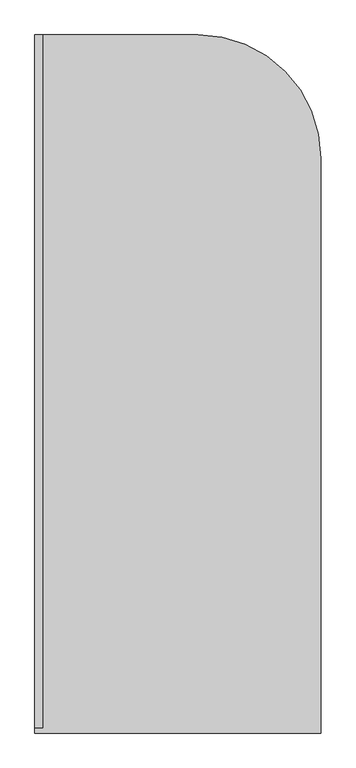
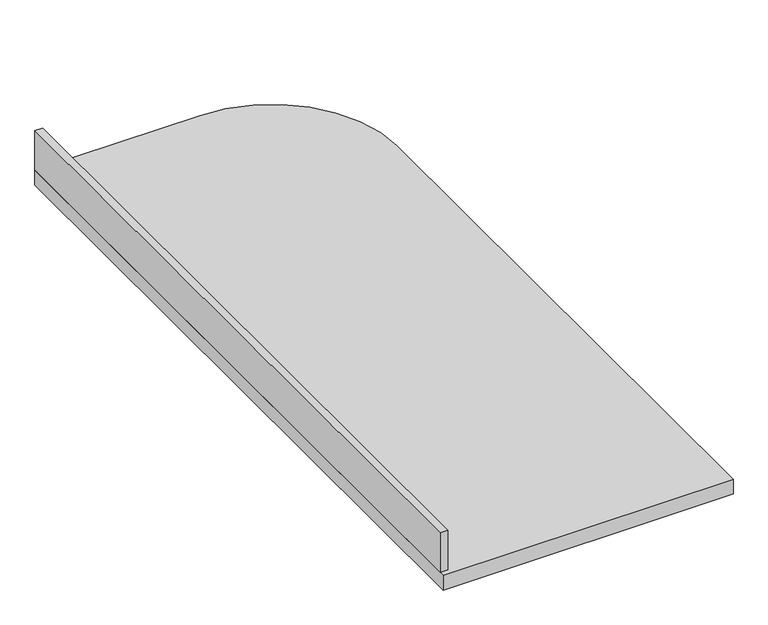
"""IFC4 building model written with IfcOpenShell, lengths in millimetres: furniture geometry, Kitchen - Baking counter : Kitchen - Baking counter."""

import ifcopenshell
import ifcopenshell.guid

model = None  # the IFC model being written
_history = None  # IfcOwnerHistory: only IFC2X3 demands one
_inside = {}  # id of a spatial element -> (the spatial element, [elements in it])
_under = {}  # id of a project, library or spatial element -> (it, [spatial elements below it])
_declared = {}  # id of a project -> (the project, [libraries it declares])
_typed = {}  # id of a type object -> (the type object, [elements of that type])
_made_of = {}  # id of a material, layer set ... -> (it, [elements and type objects made of it])


def new_model(schema):
    """Start an empty IFC model of exactly this schema.

    Asked for "IFC4X3", IfcOpenShell would pick the latest addendum, in which some entities
    have other attributes; the version numbers below select the first issue.
    IFC2X3 requires an IfcOwnerHistory on every rooted entity: one is made here for all.
    """
    global model, _history
    if schema == "IFC4X3":
        model = ifcopenshell.file(schema_version=(4, 3, 0, 0))
    else:
        model = ifcopenshell.file(schema=schema)
    _inside.clear()
    _under.clear()
    _declared.clear()
    _typed.clear()
    _made_of.clear()
    _history = None
    if model.schema == "IFC2X3":
        org = make("IfcOrganization", Name="unknown")
        user = make(
            "IfcPersonAndOrganization",
            ThePerson=make("IfcPerson", FamilyName="unknown"),
            TheOrganization=org,
        )
        app = make(
            "IfcApplication",
            ApplicationDeveloper=org,
            Version="unknown",
            ApplicationFullName="unknown",
            ApplicationIdentifier="unknown",
        )
        _history = make(
            "IfcOwnerHistory",
            OwningUser=user,
            OwningApplication=app,
            ChangeAction="ADDED",
            CreationDate=0,
        )
    return model


def make(cls, **values):
    """One entity of the class cls with the attributes given. An attribute that is None is left unset."""
    return model.create_entity(
        cls, **{name: value for name, value in values.items() if value is not None}
    )


def rooted(cls, **values):
    """An entity with a GlobalId (a new one), such as an element, a storey or a relation."""
    return make(cls, GlobalId=ifcopenshell.guid.new(), OwnerHistory=_history, **values)


def si_unit(unit_type, name, prefix=None):
    """IfcSIUnit, for example si_unit("LENGTHUNIT", "METRE", prefix="MILLI")."""
    return make("IfcSIUnit", UnitType=unit_type, Prefix=prefix, Name=name)


def assignment(units):
    """IfcUnitAssignment: the units of a project."""
    return None if units is None else make("IfcUnitAssignment", Units=units)


def point(xyz):
    """IfcCartesianPoint."""
    return None if xyz is None else make("IfcCartesianPoint", Coordinates=xyz)


def direction(xyz):
    """IfcDirection."""
    return None if xyz is None else make("IfcDirection", DirectionRatios=xyz)


def frame(location, z_axis=None, x_axis=None):
    """IfcAxis2Placement3D, a coordinate frame: its origin and axes. An axis left out is left unset."""
    return make(
        "IfcAxis2Placement3D",
        Location=point(location),
        Axis=direction(z_axis),
        RefDirection=direction(x_axis),
    )


def frame_2d(location, x_axis=None):
    """IfcAxis2Placement2D, a coordinate frame in the plane: its origin and x axis."""
    return make(
        "IfcAxis2Placement2D", Location=point(location), RefDirection=direction(x_axis)
    )


def origin():
    """The frame at (0, 0, 0) with its axes left unset."""
    return frame((0.0, 0.0, 0.0))


def place(relative_to, where):
    """IfcLocalPlacement: puts the frame where relative to a parent placement (None: the world)."""
    return make(
        "IfcLocalPlacement", PlacementRelTo=relative_to, RelativePlacement=where
    )


def context(
    kind, dimensions, precision=None, world=None, true_north=None, identifier=None
):
    """IfcGeometricRepresentationContext, for example the 3D "Model" context."""
    return make(
        "IfcGeometricRepresentationContext",
        ContextIdentifier=identifier,
        ContextType=kind,
        CoordinateSpaceDimension=dimensions,
        Precision=precision,
        WorldCoordinateSystem=world,
        TrueNorth=true_north,
    )


def project(units=None, contexts=None):
    """IfcProject with its units and contexts."""
    return rooted(
        "IfcProject",
        Name="project",
        RepresentationContexts=contexts,
        UnitsInContext=assignment(units),
    )


def spatial(cls, under=None, at=None, **own):
    """A site, building, storey or space (cls), placed at a placement, below another one or the project."""
    s = rooted(cls, ObjectPlacement=at, **own)
    if under is not None:
        _under.setdefault(under.id(), (under, []))[1].append(s)
    return s


def polyline(points):
    """IfcPolyline through the points."""
    return make("IfcPolyline", Points=[point(p) for p in points])


def circle_curve(where, radius):
    """IfcCircle in the frame where."""
    return make("IfcCircle", Position=where, Radius=radius)


def trimmed(basis, trim1, trim2, sense, master):
    """IfcTrimmedCurve: the piece of a basis curve between two trims."""
    return make(
        "IfcTrimmedCurve",
        BasisCurve=basis,
        Trim1=trim1,
        Trim2=trim2,
        SenseAgreement=sense,
        MasterRepresentation=master,
    )


def segment(curve, same_sense, transition):
    """IfcCompositeCurveSegment."""
    return make(
        "IfcCompositeCurveSegment",
        Transition=transition,
        SameSense=same_sense,
        ParentCurve=curve,
    )


def composite_curve(segments, self_intersect=None):
    """IfcCompositeCurve: segments joined end to end."""
    return make("IfcCompositeCurve", Segments=segments, SelfIntersect=self_intersect)


def outline(outer, holes=None, kind="AREA"):
    """IfcArbitraryClosedProfileDef: a profile drawn as a closed curve; with holes, ...WithVoids."""
    if holes is None:
        return make("IfcArbitraryClosedProfileDef", ProfileType=kind, OuterCurve=outer)
    return make(
        "IfcArbitraryProfileDefWithVoids",
        ProfileType=kind,
        OuterCurve=outer,
        InnerCurves=holes,
    )


def extrude(swept, where, along, depth):
    """IfcExtrudedAreaSolid: the profile swept, set in the frame where, extruded along a direction by depth."""
    return make(
        "IfcExtrudedAreaSolid",
        SweptArea=swept,
        Position=where,
        ExtrudedDirection=direction(along),
        Depth=depth,
    )


def shape(context_of_items, identifier, shape_type, items):
    """IfcShapeRepresentation: the items that make up one representation, for example the "Body"."""
    return make(
        "IfcShapeRepresentation",
        ContextOfItems=context_of_items,
        RepresentationIdentifier=identifier,
        RepresentationType=shape_type,
        Items=items,
    )


def source(mapping_origin, context_of_items, identifier, shape_type, items):
    """IfcRepresentationMap: a shape defined once, which mapped items show again and again."""
    return make(
        "IfcRepresentationMap",
        MappingOrigin=mapping_origin,
        MappedRepresentation=shape(context_of_items, identifier, shape_type, items),
    )


def transform(
    local_origin,
    x_axis=None,
    y_axis=None,
    z_axis=None,
    scale=None,
    scale2=None,
    scale3=None,
    uniform=True,
):
    """IfcCartesianTransformationOperator3D, or its non-uniform kind. x_axis, y_axis, z_axis: its Axis1, 2, 3."""
    if uniform:
        return make(
            "IfcCartesianTransformationOperator3D",
            Axis1=direction(x_axis),
            Axis2=direction(y_axis),
            LocalOrigin=point(local_origin),
            Scale=scale,
            Axis3=direction(z_axis),
        )
    return make(
        "IfcCartesianTransformationOperator3DnonUniform",
        Axis1=direction(x_axis),
        Axis2=direction(y_axis),
        LocalOrigin=point(local_origin),
        Scale=scale,
        Axis3=direction(z_axis),
        Scale2=scale2,
        Scale3=scale3,
    )


def mapped(mapping_source, mapping_target):
    """IfcMappedItem: shows the shape of a source again, moved by a transform."""
    return make(
        "IfcMappedItem", MappingSource=mapping_source, MappingTarget=mapping_target
    )


def made_of(thing, what):
    """Note that an element or type object is made of a material, layer set ...; save() writes the relation."""
    if what is not None:
        _made_of.setdefault(what.id(), (what, []))[1].append(thing)
    return thing


def element(
    cls,
    number,
    at=None,
    inside=None,
    cuts=None,
    type_object=None,
    material=None,
    context=None,
    identifier="Body",
    shape_type=None,
    held_by="IfcProductDefinitionShape",
    body=None,
    shapes=None,
    **own,
):
    """One element of the class cls, such as IfcWall. Its Tag is "e" and its number.

    at: its placement. inside: the storey or other place that contains it. cuts: it is an
    opening in that element (IfcRelVoidsElement). A single representation is given by context,
    identifier, shape_type and body (its items); several are given by shapes. held_by: the class
    of the entity that holds the representations. save() writes the other relations.
    """
    e = rooted(cls, Tag="e%d" % number, ObjectPlacement=at, **own)
    if body is not None:
        shapes = [shape(context, identifier, shape_type, body)]
    if shapes is not None:
        e.Representation = make(held_by, Representations=shapes)
    if inside is not None:
        _inside.setdefault(inside.id(), (inside, []))[1].append(e)
    if cuts is not None:
        rooted(
            "IfcRelVoidsElement", RelatingBuildingElement=cuts, RelatedOpeningElement=e
        )
    if type_object is not None:
        _typed.setdefault(type_object.id(), (type_object, []))[1].append(e)
    return made_of(e, material)


def aggregate(whole, parts):
    """IfcRelAggregates: a whole, such as a stair, and the parts it consists of."""
    return rooted("IfcRelAggregates", RelatingObject=whole, RelatedObjects=parts)


def save(model, path):
    """Write the relations noted so far, then the file.

    IfcRelAggregates (storeys below a building ...), IfcRelContainedInSpatialStructure (elements
    in a storey), IfcRelDefinesByType, IfcRelAssociatesMaterial and IfcRelDeclares: one each for
    every whole, place, type object, material and project.
    """
    for whole, parts in _under.values():
        aggregate(whole, parts)
    for where, things in _inside.values():
        rooted(
            "IfcRelContainedInSpatialStructure",
            RelatedElements=things,
            RelatingStructure=where,
        )
    for kind, things in _typed.values():
        rooted("IfcRelDefinesByType", RelatedObjects=things, RelatingType=kind)
    for what, things in _made_of.values():
        rooted("IfcRelAssociatesMaterial", RelatedObjects=things, RelatingMaterial=what)
    for by, libraries in _declared.values():
        rooted("IfcRelDeclares", RelatingContext=by, RelatedDefinitions=libraries)
    model.write(path)


def furniture_77338e29(model_context):
    return source(origin(), model_context, "Body", "SweptSolid", [
        extrude(outline(polyline([(3765.55, 10655.3), (3765.55, 12369.8), (3784.6, 12369.8), (3784.6, 10655.3), (3765.55, 10655.3)])), frame((0.0, 0.0, 914.4), z_axis=(0.0, 0.0, 1.0), x_axis=(1.0, 0.0, 0.0)), (0.0, 0.0, 1.0), 101.6),
        extrude(outline(composite_curve([segment(polyline([(4474.1779098, 12065.0), (4474.1779098, 10642.6), (3765.55, 10642.6), (3765.55, 12369.8), (4169.3779098, 12369.8)]), True, "CONTINUOUS"), segment(trimmed(circle_curve(frame_2d((4169.3779098, 12065.0)), 304.8), [point((4169.3779098, 12369.8))], [point((4474.1779098, 12065.0))], False, "CARTESIAN"), True, "CONTINUOUS")], self_intersect=False)), frame((0.0, 0.0, 876.3), z_axis=(0.0, 0.0, 1.0), x_axis=(1.0, 0.0, 0.0)), (0.0, 0.0, 1.0), 38.1),
    ])


if __name__ == "__main__":
    model = new_model("IFC4")
    model_context = context("Model", 3, world=origin())
    ifc_project = project(units=[si_unit("LENGTHUNIT", "METRE", prefix="MILLI")], contexts=[model_context])
    site = spatial("IfcSite", under=ifc_project)
    building = spatial("IfcBuilding", under=site)
    placement = place(None, origin())
    furniture_shape = furniture_77338e29(model_context)
    element("IfcFurniture", 1, ObjectType="Kitchen - Baking counter : Kitchen - Baking counter", at=placement, inside=building, context=model_context, shape_type="MappedRepresentation", body=[
        mapped(furniture_shape, transform((0.0, 0.0, 0.0), x_axis=(1.0, 0.0, 0.0), y_axis=(0.0, 1.0, 0.0), z_axis=(0.0, 0.0, 1.0))),
    ])
    save(model, "model.ifc")

# Revit data of these elements
# Type "Kitchen - Baking counter : Kitchen - Baking counter"
#   COBie.Type = no
# Element 1 (IfcFurniture, "Kitchen - Baking counter : Kitchen - Baking counter")
#   Materials on its faces: "Corian - Dusk"
# Materials
#   "Corian - Dusk": class "Plastic", colour RGB 75 95 146, transparency 0, Manufacturer = "Corning", Cost = 0
